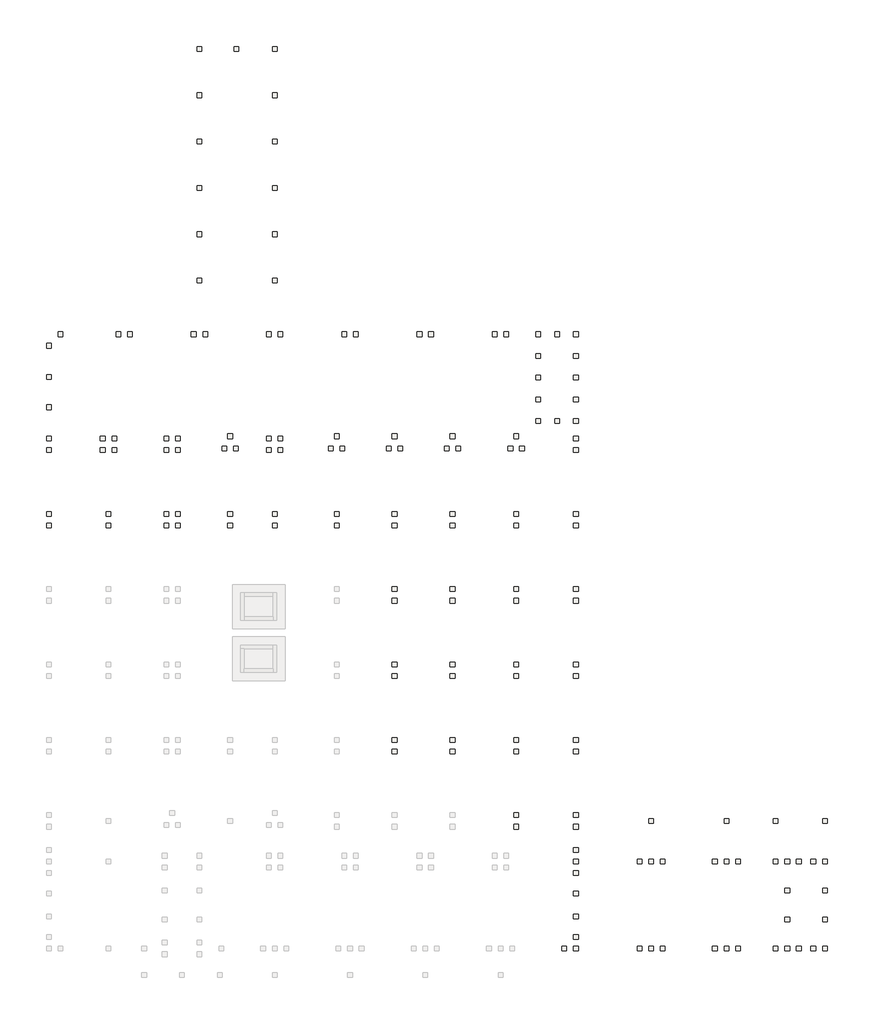
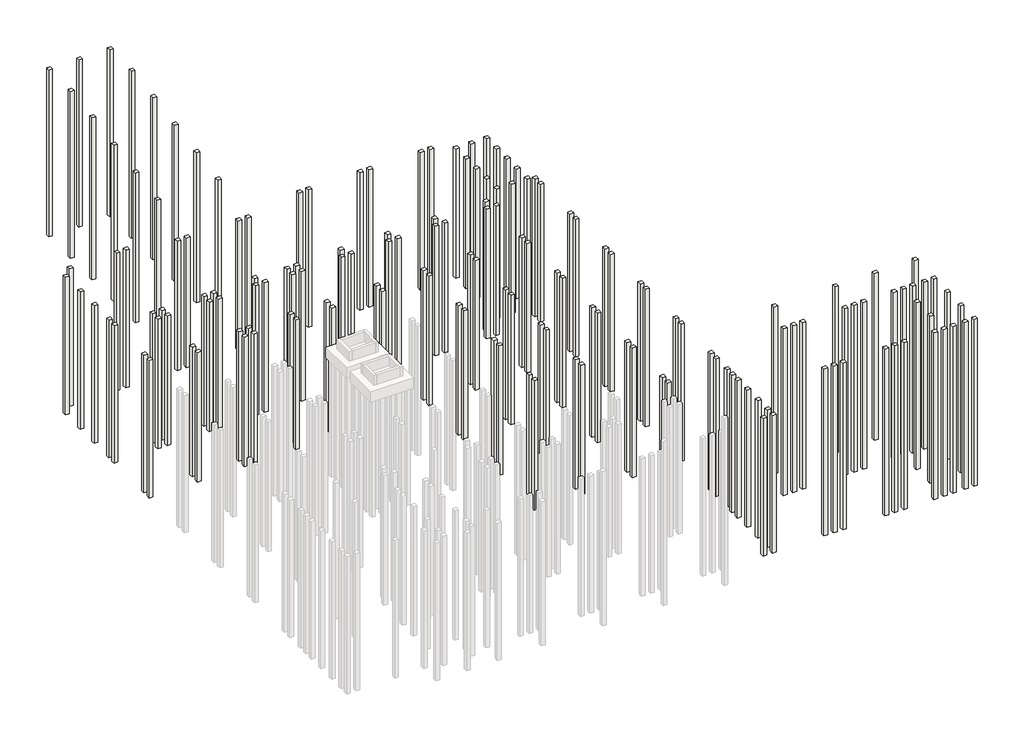
# Not in any storey, part 2 of 2: 160 slabs.
# Revit data of these elements (continued)
# Element 105 (IfcSlab, "NLRS_17_SFO_TLB_funderingspaal geheid beton prefab-AV-MMBPC_gen_rsf : heipaal beton prefab_gen__bxh 400x400")
#   IfcGUID = "3loy75XKz2Rw4dS8JWiatE"
#   Slanted Angle = 0.00°
#   NLRS_S_draagvermogen_trek = 0.00 kN
#   NLRS_S_draagvermogen_druk = 0.00 kN
#   Angle = 0.00°
#   IsExternal = yes
#   LoadBearing = yes
#   Slanted = 0
#   Phase Created = NLRS_nieuw
#   Materials on its faces: "NLRS_f2_beton prefab_gen_rsf"
# Element 106 (IfcSlab, "NLRS_17_SFO_TLB_funderingspaal geheid beton prefab-AV-MMBPC_gen_rsf : heipaal beton prefab_gen__bxh 400x400")
#   IfcGUID = "3loy75XKz2Rw4dS8JWiatC"
#   Slanted Angle = 0.00°
#   NLRS_S_draagvermogen_trek = 0.00 kN
#   NLRS_S_draagvermogen_druk = 0.00 kN
#   Angle = 0.00°
#   IsExternal = yes
#   LoadBearing = yes
#   Slanted = 0
#   Phase Created = NLRS_nieuw
#   Materials on its faces: "NLRS_f2_beton prefab_gen_rsf"
# Element 107 (IfcSlab, "NLRS_17_SFO_TLB_funderingspaal geheid beton prefab-AV-MMBPC_gen_rsf : heipaal beton prefab_gen__bxh 400x400")
#   IfcGUID = "3loy75XKz2Rw4dS8JWiatv"
#   Slanted Angle = 0.00°
#   NLRS_S_draagvermogen_trek = 0.00 kN
#   NLRS_S_draagvermogen_druk = 0.00 kN
#   Angle = 0.00°
#   IsExternal = yes
#   LoadBearing = yes
#   Slanted = 0
#   Phase Created = NLRS_nieuw
#   Materials on its faces: "NLRS_f2_beton prefab_gen_rsf"
# Element 108 (IfcSlab, "NLRS_17_SFO_TLB_funderingspaal geheid beton prefab-AV-MMBPC_gen_rsf : heipaal beton prefab_gen__bxh 400x400")
#   IfcGUID = "3loy75XKz2Rw4dS8JWiat$"
#   Slanted Angle = 0.00°
#   NLRS_S_draagvermogen_trek = 0.00 kN
#   NLRS_S_draagvermogen_druk = 0.00 kN
#   Angle = 0.00°
#   IsExternal = yes
#   LoadBearing = yes
#   Slanted = 0
#   Phase Created = NLRS_nieuw
#   Materials on its faces: "NLRS_f2_beton prefab_gen_rsf"
# Element 109 (IfcSlab, "NLRS_17_SFO_TLB_funderingspaal geheid beton prefab-AV-MMBPC_gen_rsf : heipaal beton prefab_gen__bxh 400x400")
#   IfcGUID = "3loy75XKz2Rw4dS8JWiaEQ"
#   Slanted Angle = 0.00°
#   NLRS_S_draagvermogen_trek = 0.00 kN
#   NLRS_S_draagvermogen_druk = 0.00 kN
#   Angle = 0.00°
#   IsExternal = yes
#   LoadBearing = yes
#   Slanted = 0
#   Phase Created = NLRS_nieuw
#   Materials on its faces: "NLRS_f2_beton prefab_gen_rsf"
# Element 110 (IfcSlab, "NLRS_17_SFO_TLB_funderingspaal geheid beton prefab-AV-MMBPC_gen_rsf : heipaal beton prefab_gen__bxh 400x400")
#   IfcGUID = "3loy75XKz2Rw4dS8JWiaEW"
#   Slanted Angle = 0.00°
#   NLRS_S_draagvermogen_trek = 0.00 kN
#   NLRS_S_draagvermogen_druk = 0.00 kN
#   Angle = 0.00°
#   IsExternal = yes
#   LoadBearing = yes
#   Slanted = 0
#   Phase Created = NLRS_nieuw
#   Materials on its faces: "NLRS_f2_beton prefab_gen_rsf"
# Element 111 (IfcSlab, "NLRS_17_SFO_TLB_funderingspaal geheid beton prefab-AV-MMBPC_gen_rsf : heipaal beton prefab_gen__bxh 400x400")
#   IfcGUID = "3loy75XKz2Rw4dS8JWia10"
#   Slanted Angle = 0.00°
#   NLRS_S_draagvermogen_trek = 0.00 kN
#   NLRS_S_draagvermogen_druk = 0.00 kN
#   Angle = 0.00°
#   IsExternal = yes
#   LoadBearing = yes
#   Slanted = 0
#   Phase Created = NLRS_nieuw
#   Materials on its faces: "NLRS_f2_beton prefab_gen_rsf"
# Element 112 (IfcSlab, "NLRS_17_SFO_TLB_funderingspaal geheid beton prefab-AV-MMBPC_gen_rsf : heipaal beton prefab_gen__bxh 400x400")
#   IfcGUID = "3loy75XKz2Rw4dS8JWia16"
#   Slanted Angle = 0.00°
#   NLRS_S_draagvermogen_trek = 0.00 kN
#   NLRS_S_draagvermogen_druk = 0.00 kN
#   Angle = 0.00°
#   IsExternal = yes
#   LoadBearing = yes
#   Slanted = 0
#   Phase Created = NLRS_nieuw
#   Materials on its faces: "NLRS_f2_beton prefab_gen_rsf"
# Element 113 (IfcSlab, "NLRS_17_SFO_TLB_funderingspaal geheid beton prefab-AV-MMBPC_gen_rsf : heipaal beton prefab_gen__bxh 400x400")
#   IfcGUID = "3loy75XKz2Rw4dS8JWia1p"
#   Slanted Angle = 0.00°
#   NLRS_S_draagvermogen_trek = 0.00 kN
#   NLRS_S_draagvermogen_druk = 0.00 kN
#   Angle = 0.00°
#   IsExternal = yes
#   LoadBearing = yes
#   Slanted = 0
#   Phase Created = NLRS_nieuw
#   Materials on its faces: "NLRS_f2_beton prefab_gen_rsf"
# Element 114 (IfcSlab, "NLRS_17_SFO_TLB_funderingspaal geheid beton prefab-AV-MMBPC_gen_rsf : heipaal beton prefab_gen__bxh 400x400")
#   IfcGUID = "3loy75XKz2Rw4dS8JWia1n"
#   Slanted Angle = 0.00°
#   NLRS_S_draagvermogen_trek = 0.00 kN
#   NLRS_S_draagvermogen_druk = 0.00 kN
#   Angle = 0.00°
#   IsExternal = yes
#   LoadBearing = yes
#   Slanted = 0
#   Phase Created = NLRS_nieuw
#   Materials on its faces: "NLRS_f2_beton prefab_gen_rsf"
# Element 115 (IfcSlab, "NLRS_17_SFO_TLB_funderingspaal geheid beton prefab-AV-MMBPC_gen_rsf : heipaal beton prefab_gen__bxh 400x400")
#   IfcGUID = "3loy75XKz2Rw4dS8JWia5x"
#   Slanted Angle = 0.00°
#   NLRS_S_draagvermogen_trek = 0.00 kN
#   NLRS_S_draagvermogen_druk = 0.00 kN
#   Angle = 0.00°
#   IsExternal = yes
#   LoadBearing = yes
#   Slanted = 0
#   Phase Created = NLRS_nieuw
#   Materials on its faces: "NLRS_f2_beton prefab_gen_rsf"
# Element 116 (IfcSlab, "NLRS_17_SFO_TLB_funderingspaal geheid beton prefab-AV-MMBPC_gen_rsf : heipaal beton prefab_gen__bxh 400x400")
#   IfcGUID = "3loy75XKz2Rw4dS8JWia4Y"
#   Slanted Angle = 0.00°
#   NLRS_S_draagvermogen_trek = 0.00 kN
#   NLRS_S_draagvermogen_druk = 0.00 kN
#   Angle = 0.00°
#   IsExternal = yes
#   LoadBearing = yes
#   Slanted = 0
#   Phase Created = NLRS_nieuw
#   Materials on its faces: "NLRS_f2_beton prefab_gen_rsf"
# Element 117 (IfcSlab, "NLRS_17_SFO_TLB_funderingspaal geheid beton prefab-AV-MMBPC_gen_rsf : heipaal beton prefab_gen__bxh 400x400")
#   IfcGUID = "3loy75XKz2Rw4dS8JWia4W"
#   Slanted Angle = 0.00°
#   NLRS_S_draagvermogen_trek = 0.00 kN
#   NLRS_S_draagvermogen_druk = 0.00 kN
#   Angle = 0.00°
#   IsExternal = yes
#   LoadBearing = yes
#   Slanted = 0
#   Phase Created = NLRS_nieuw
#   Materials on its faces: "NLRS_f2_beton prefab_gen_rsf"
# Element 118 (IfcSlab, "NLRS_17_SFO_TLB_funderingspaal geheid beton prefab-AV-MMBPC_gen_rsf : heipaal beton prefab_gen__bxh 400x400")
#   IfcGUID = "1JrsWFyZX6xPuD52juGVxa"
#   Slanted Angle = 0.00°
#   NLRS_S_draagvermogen_trek = 0.00 kN
#   NLRS_S_draagvermogen_druk = 0.00 kN
#   Angle = 0.00°
#   IsExternal = yes
#   LoadBearing = yes
#   Slanted = 0
#   Phase Created = NLRS_nieuw
#   Materials on its faces: "NLRS_f2_beton prefab_gen_rsf"
# Element 119 (IfcSlab, "NLRS_17_SFO_TLB_funderingspaal geheid beton prefab-AV-MMBPC_gen_rsf : heipaal beton prefab_gen__bxh 400x400")
#   IfcGUID = "1JrsWFyZX6xPuD52juGVvn"
#   Slanted Angle = 0.00°
#   NLRS_S_draagvermogen_trek = 0.00 kN
#   NLRS_S_draagvermogen_druk = 0.00 kN
#   Angle = 0.00°
#   IsExternal = yes
#   LoadBearing = yes
#   Slanted = 0
#   Phase Created = NLRS_nieuw
#   Materials on its faces: "NLRS_f2_beton prefab_gen_rsf"
# Element 120 (IfcSlab, "NLRS_17_SFO_TLB_funderingspaal geheid beton prefab-AV-MMBPC_gen_rsf : heipaal beton prefab_gen__bxh 400x400")
#   IfcGUID = "1JrsWFyZX6xPuD52juGVv2"
#   Slanted Angle = 0.00°
#   NLRS_S_draagvermogen_trek = 0.00 kN
#   NLRS_S_draagvermogen_druk = 0.00 kN
#   Angle = 0.00°
#   IsExternal = yes
#   LoadBearing = yes
#   Slanted = 0
#   Phase Created = NLRS_nieuw
#   Materials on its faces: "NLRS_f2_beton prefab_gen_rsf"
# Element 121 (IfcSlab, "NLRS_17_SFO_TLB_funderingspaal geheid beton prefab-AV-MMBPC_gen_rsf : heipaal beton prefab_gen__bxh 400x400")
#   IfcGUID = "1JrsWFyZX6xPuD52juGV_f"
#   Slanted Angle = 0.00°
#   NLRS_S_draagvermogen_trek = 0.00 kN
#   NLRS_S_draagvermogen_druk = 0.00 kN
#   Angle = 0.00°
#   IsExternal = yes
#   LoadBearing = yes
#   Slanted = 0
#   Phase Created = NLRS_nieuw
#   Materials on its faces: "NLRS_f2_beton prefab_gen_rsf"
# Element 122 (IfcSlab, "NLRS_17_SFO_TLB_funderingspaal geheid beton prefab-AV-MMBPC_gen_rsf : heipaal beton prefab_gen__bxh 400x400")
#   IfcGUID = "1JrsWFyZX6xPuD52juGV_d"
#   Slanted Angle = 0.00°
#   NLRS_S_draagvermogen_trek = 0.00 kN
#   NLRS_S_draagvermogen_druk = 0.00 kN
#   Angle = 0.00°
#   IsExternal = yes
#   LoadBearing = yes
#   Slanted = 0
#   Phase Created = NLRS_nieuw
#   Materials on its faces: "NLRS_f2_beton prefab_gen_rsf"
# Element 123 (IfcSlab, "NLRS_17_SFO_TLB_funderingspaal geheid beton prefab-AV-MMBPC_gen_rsf : heipaal beton prefab_gen__bxh 400x400")
#   IfcGUID = "1JrsWFyZX6xPuD52juGV_b"
#   Slanted Angle = 0.00°
#   NLRS_S_draagvermogen_trek = 0.00 kN
#   NLRS_S_draagvermogen_druk = 0.00 kN
#   Angle = 0.00°
#   IsExternal = yes
#   LoadBearing = yes
#   Slanted = 0
#   Phase Created = NLRS_nieuw
#   Materials on its faces: "NLRS_f2_beton prefab_gen_rsf"
# Element 124 (IfcSlab, "NLRS_17_SFO_TLB_funderingspaal geheid beton prefab-AV-MMBPC_gen_rsf : heipaal beton prefab_gen__bxh 400x400")
#   IfcGUID = "1JrsWFyZX6xPuD52juGV_G"
#   Slanted Angle = 0.00°
#   NLRS_S_draagvermogen_trek = 0.00 kN
#   NLRS_S_draagvermogen_druk = 0.00 kN
#   Angle = 0.00°
#   IsExternal = yes
#   LoadBearing = yes
#   Slanted = 0
#   Phase Created = NLRS_nieuw
#   Materials on its faces: "NLRS_f2_beton prefab_gen_rsf"
# Element 125 (IfcSlab, "NLRS_17_SFO_TLB_funderingspaal geheid beton prefab-AV-MMBPC_gen_rsf : heipaal beton prefab_gen__bxh 400x400")
#   IfcGUID = "1JrsWFyZX6xPuD52juGV_E"
#   Slanted Angle = 0.00°
#   NLRS_S_draagvermogen_trek = 0.00 kN
#   NLRS_S_draagvermogen_druk = 0.00 kN
#   Angle = 0.00°
#   IsExternal = yes
#   LoadBearing = yes
#   Slanted = 0
#   Phase Created = NLRS_nieuw
#   Materials on its faces: "NLRS_f2_beton prefab_gen_rsf"
# Element 126 (IfcSlab, "NLRS_17_SFO_TLB_funderingspaal geheid beton prefab-AV-MMBPC_gen_rsf : heipaal beton prefab_gen__bxh 400x400")
#   IfcGUID = "1JrsWFyZX6xPuD52juGV_C"
#   Slanted Angle = 0.00°
#   NLRS_S_draagvermogen_trek = 0.00 kN
#   NLRS_S_draagvermogen_druk = 0.00 kN
#   Angle = 0.00°
#   IsExternal = yes
#   LoadBearing = yes
#   Slanted = 0
#   Phase Created = NLRS_nieuw
#   Materials on its faces: "NLRS_f2_beton prefab_gen_rsf"
# Element 127 (IfcSlab, "NLRS_17_SFO_TLB_funderingspaal geheid beton prefab-AV-MMBPC_gen_rsf : heipaal beton prefab_gen__bxh 400x400")
#   IfcGUID = "1JrsWFyZX6xPuD52juGV_A"
#   Slanted Angle = 0.00°
#   NLRS_S_draagvermogen_trek = 0.00 kN
#   NLRS_S_draagvermogen_druk = 0.00 kN
#   Angle = 0.00°
#   IsExternal = yes
#   LoadBearing = yes
#   Slanted = 0
#   Phase Created = NLRS_nieuw
#   Materials on its faces: "NLRS_f2_beton prefab_gen_rsf"
# Element 128 (IfcSlab, "NLRS_17_SFO_TLB_funderingspaal geheid beton prefab-AV-MMBPC_gen_rsf : heipaal beton prefab_gen__bxh 400x400")
#   IfcGUID = "1JrsWFyZX6xPuD52juGV_8"
#   Slanted Angle = 0.00°
#   NLRS_S_draagvermogen_trek = 0.00 kN
#   NLRS_S_draagvermogen_druk = 0.00 kN
#   Angle = 0.00°
#   IsExternal = yes
#   LoadBearing = yes
#   Slanted = 0
#   Phase Created = NLRS_nieuw
#   Materials on its faces: "NLRS_f2_beton prefab_gen_rsf"
# Element 129 (IfcSlab, "NLRS_17_SFO_TLB_funderingspaal geheid beton prefab-AV-MMBPC_gen_rsf : heipaal beton prefab_gen__bxh 400x400")
#   IfcGUID = "1JrsWFyZX6xPuD52juGV_6"
#   Slanted Angle = 0.00°
#   NLRS_S_draagvermogen_trek = 0.00 kN
#   NLRS_S_draagvermogen_druk = 0.00 kN
#   Angle = 0.00°
#   IsExternal = yes
#   LoadBearing = yes
#   Slanted = 0
#   Phase Created = NLRS_nieuw
#   Materials on its faces: "NLRS_f2_beton prefab_gen_rsf"
# Element 130 (IfcSlab, "NLRS_17_SFO_TLB_funderingspaal geheid beton prefab-AV-MMBPC_gen_rsf : heipaal beton prefab_gen__bxh 400x400")
#   IfcGUID = "1JrsWFyZX6xPuD52juGV$T"
#   Slanted Angle = 0.00°
#   NLRS_S_draagvermogen_trek = 0.00 kN
#   NLRS_S_draagvermogen_druk = 0.00 kN
#   Angle = 0.00°
#   IsExternal = yes
#   LoadBearing = yes
#   Slanted = 0
#   Phase Created = NLRS_nieuw
#   Materials on its faces: "NLRS_f2_beton prefab_gen_rsf"
# Element 131 (IfcSlab, "NLRS_17_SFO_TLB_funderingspaal geheid beton prefab-AV-MMBPC_gen_rsf : heipaal beton prefab_gen__bxh 400x400")
#   IfcGUID = "1JrsWFyZX6xPuD52juGV$G"
#   Slanted Angle = 0.00°
#   NLRS_S_draagvermogen_trek = 0.00 kN
#   NLRS_S_draagvermogen_druk = 0.00 kN
#   Angle = 0.00°
#   IsExternal = yes
#   LoadBearing = yes
#   Slanted = 0
#   Phase Created = NLRS_nieuw
#   Materials on its faces: "NLRS_f2_beton prefab_gen_rsf"
# Element 132 (IfcSlab, "NLRS_17_SFO_TLB_funderingspaal geheid beton prefab-AV-MMBPC_gen_rsf : heipaal beton prefab_gen__bxh 400x400")
#   IfcGUID = "1JrsWFyZX6xPuD52juGVyj"
#   Slanted Angle = 0.00°
#   NLRS_S_draagvermogen_trek = 0.00 kN
#   NLRS_S_draagvermogen_druk = 0.00 kN
#   Angle = 0.00°
#   IsExternal = yes
#   LoadBearing = yes
#   Slanted = 0
#   Phase Created = NLRS_nieuw
#   Materials on its faces: "NLRS_f2_beton prefab_gen_rsf"
# Element 133 (IfcSlab, "NLRS_17_SFO_TLB_funderingspaal geheid beton prefab-AV-MMBPC_gen_rsf : heipaal beton prefab_gen__bxh 400x400")
#   IfcGUID = "1JrsWFyZX6xPuD52juGVy1"
#   Slanted Angle = 0.00°
#   NLRS_S_draagvermogen_trek = 0.00 kN
#   NLRS_S_draagvermogen_druk = 0.00 kN
#   Angle = 0.00°
#   IsExternal = yes
#   LoadBearing = yes
#   Slanted = 0
#   Phase Created = NLRS_nieuw
#   Materials on its faces: "NLRS_f2_beton prefab_gen_rsf"
# Element 134 (IfcSlab, "NLRS_17_SFO_TLB_funderingspaal geheid beton prefab-AV-MMBPC_gen_rsf : heipaal beton prefab_gen__bxh 400x400")
#   IfcGUID = "1JrsWFyZX6xPuD52juGVz$"
#   Slanted Angle = 0.00°
#   NLRS_S_draagvermogen_trek = 0.00 kN
#   NLRS_S_draagvermogen_druk = 0.00 kN
#   Angle = 0.00°
#   IsExternal = yes
#   LoadBearing = yes
#   Slanted = 0
#   Phase Created = NLRS_nieuw
#   Materials on its faces: "NLRS_f2_beton prefab_gen_rsf"
# Element 135 (IfcSlab, "NLRS_17_SFO_TLB_funderingspaal geheid beton prefab-AV-MMBPC_gen_rsf : heipaal beton prefab_gen__bxh 400x400")
#   IfcGUID = "1JrsWFyZX6xPuD52juGVzz"
#   Slanted Angle = 0.00°
#   NLRS_S_draagvermogen_trek = 0.00 kN
#   NLRS_S_draagvermogen_druk = 0.00 kN
#   Angle = 0.00°
#   IsExternal = yes
#   LoadBearing = yes
#   Slanted = 0
#   Phase Created = NLRS_nieuw
#   Materials on its faces: "NLRS_f2_beton prefab_gen_rsf"
# Element 136 (IfcSlab, "NLRS_17_SFO_TLB_funderingspaal geheid beton prefab-AV-MMBPC_gen_rsf : heipaal beton prefab_gen__bxh 400x400")
#   IfcGUID = "1JrsWFyZX6xPuD52juGVzI"
#   Slanted Angle = 0.00°
#   NLRS_S_draagvermogen_trek = 0.00 kN
#   NLRS_S_draagvermogen_druk = 0.00 kN
#   Angle = 0.00°
#   IsExternal = yes
#   LoadBearing = yes
#   Slanted = 0
#   Phase Created = NLRS_nieuw
#   Materials on its faces: "NLRS_f2_beton prefab_gen_rsf"
# Element 137 (IfcSlab, "NLRS_17_SFO_TLB_funderingspaal geheid beton prefab-AV-MMBPC_gen_rsf : heipaal beton prefab_gen__bxh 400x400")
#   IfcGUID = "1JrsWFyZX6xPuD52juGVz7"
#   Slanted Angle = 0.00°
#   NLRS_S_draagvermogen_trek = 0.00 kN
#   NLRS_S_draagvermogen_druk = 0.00 kN
#   Angle = 0.00°
#   IsExternal = yes
#   LoadBearing = yes
#   Slanted = 0
#   Phase Created = NLRS_nieuw
#   Materials on its faces: "NLRS_f2_beton prefab_gen_rsf"
# Element 138 (IfcSlab, "NLRS_17_SFO_TLB_funderingspaal geheid beton prefab-AV-MMBPC_gen_rsf : heipaal beton prefab_gen__bxh 400x400")
#   IfcGUID = "1JrsWFyZX6xPuD52juGVog"
#   Slanted Angle = 0.00°
#   NLRS_S_draagvermogen_trek = 0.00 kN
#   NLRS_S_draagvermogen_druk = 0.00 kN
#   Angle = 0.00°
#   IsExternal = yes
#   LoadBearing = yes
#   Slanted = 0
#   Phase Created = NLRS_nieuw
#   Materials on its faces: "NLRS_f2_beton prefab_gen_rsf"
# Element 139 (IfcSlab, "NLRS_17_SFO_TLB_funderingspaal geheid beton prefab-AV-MMBPC_gen_rsf : heipaal beton prefab_gen__bxh 400x400")
#   IfcGUID = "1JrsWFyZX6xPuD52juGVoe"
#   Slanted Angle = 0.00°
#   NLRS_S_draagvermogen_trek = 0.00 kN
#   NLRS_S_draagvermogen_druk = 0.00 kN
#   Angle = 0.00°
#   IsExternal = yes
#   LoadBearing = yes
#   Slanted = 0
#   Phase Created = NLRS_nieuw
#   Materials on its faces: "NLRS_f2_beton prefab_gen_rsf"
# Element 140 (IfcSlab, "NLRS_17_SFO_TLB_funderingspaal geheid beton prefab-AV-MMBPC_gen_rsf : heipaal beton prefab_gen__bxh 400x400")
#   IfcGUID = "1JrsWFyZX6xPuD52juGVpj"
#   Slanted Angle = 0.00°
#   NLRS_S_draagvermogen_trek = 0.00 kN
#   NLRS_S_draagvermogen_druk = 0.00 kN
#   Angle = 0.00°
#   IsExternal = yes
#   LoadBearing = yes
#   Slanted = 0
#   Phase Created = NLRS_nieuw
#   Materials on its faces: "NLRS_f2_beton prefab_gen_rsf"
# Element 141 (IfcSlab, "NLRS_17_SFO_TLB_funderingspaal geheid beton prefab-AV-MMBPC_gen_rsf : heipaal beton prefab_gen__bxh 400x400")
#   IfcGUID = "1JrsWFyZX6xPuD52juGVph"
#   Slanted Angle = 0.00°
#   NLRS_S_draagvermogen_trek = 0.00 kN
#   NLRS_S_draagvermogen_druk = 0.00 kN
#   Angle = 0.00°
#   IsExternal = yes
#   LoadBearing = yes
#   Slanted = 0
#   Phase Created = NLRS_nieuw
#   Materials on its faces: "NLRS_f2_beton prefab_gen_rsf"
# Element 142 (IfcSlab, "NLRS_17_SFO_TLB_funderingspaal geheid beton prefab-AV-MMBPC_gen_rsf : heipaal beton prefab_gen__bxh 400x400")
#   IfcGUID = "1JrsWFyZX6xPuD52juGVp8"
#   Slanted Angle = 0.00°
#   NLRS_S_draagvermogen_trek = 0.00 kN
#   NLRS_S_draagvermogen_druk = 0.00 kN
#   Angle = 0.00°
#   IsExternal = yes
#   LoadBearing = yes
#   Slanted = 0
#   Phase Created = NLRS_nieuw
#   Materials on its faces: "NLRS_f2_beton prefab_gen_rsf"
# Element 143 (IfcSlab, "NLRS_17_SFO_TLB_funderingspaal geheid beton prefab-AV-MMBPC_gen_rsf : heipaal beton prefab_gen__bxh 400x400")
#   IfcGUID = "1JrsWFyZX6xPuD52juGVp6"
#   Slanted Angle = 0.00°
#   NLRS_S_draagvermogen_trek = 0.00 kN
#   NLRS_S_draagvermogen_druk = 0.00 kN
#   Angle = 0.00°
#   IsExternal = yes
#   LoadBearing = yes
#   Slanted = 0
#   Phase Created = NLRS_nieuw
#   Materials on its faces: "NLRS_f2_beton prefab_gen_rsf"
# Element 144 (IfcSlab, "NLRS_17_SFO_TLB_funderingspaal geheid beton prefab-AV-MMBPC_gen_rsf : heipaal beton prefab_gen__bxh 400x400")
#   IfcGUID = "1JrsWFyZX6xPuD52juGVmn"
#   Slanted Angle = 0.00°
#   NLRS_S_draagvermogen_trek = 0.00 kN
#   NLRS_S_draagvermogen_druk = 0.00 kN
#   Angle = 0.00°
#   IsExternal = yes
#   LoadBearing = yes
#   Slanted = 0
#   Phase Created = NLRS_nieuw
#   Materials on its faces: "NLRS_f2_beton prefab_gen_rsf"
# Element 145 (IfcSlab, "NLRS_17_SFO_TLB_funderingspaal geheid beton prefab-AV-MMBPC_gen_rsf : heipaal beton prefab_gen__bxh 400x400")
#   IfcGUID = "1JrsWFyZX6xPuD52juGVm6"
#   Slanted Angle = 0.00°
#   NLRS_S_draagvermogen_trek = 0.00 kN
#   NLRS_S_draagvermogen_druk = 0.00 kN
#   Angle = 0.00°
#   IsExternal = yes
#   LoadBearing = yes
#   Slanted = 0
#   Phase Created = NLRS_nieuw
#   Materials on its faces: "NLRS_f2_beton prefab_gen_rsf"
# Element 146 (IfcSlab, "NLRS_17_SFO_TLB_funderingspaal geheid beton prefab-AV-MMBPC_gen_rsf : heipaal beton prefab_gen__bxh 400x400")
#   IfcGUID = "1JrsWFyZX6xPuD52juGVnx"
#   Slanted Angle = 0.00°
#   NLRS_S_draagvermogen_trek = 0.00 kN
#   NLRS_S_draagvermogen_druk = 0.00 kN
#   Angle = 0.00°
#   IsExternal = yes
#   LoadBearing = yes
#   Slanted = 0
#   Phase Created = NLRS_nieuw
#   Materials on its faces: "NLRS_f2_beton prefab_gen_rsf"
# Element 147 (IfcSlab, "NLRS_17_SFO_TLB_funderingspaal geheid beton prefab-AV-MMBPC_gen_rsf : heipaal beton prefab_gen__bxh 400x400")
#   IfcGUID = "1JrsWFyZX6xPuD52juGVnv"
#   Slanted Angle = 0.00°
#   NLRS_S_draagvermogen_trek = 0.00 kN
#   NLRS_S_draagvermogen_druk = 0.00 kN
#   Angle = 0.00°
#   IsExternal = yes
#   LoadBearing = yes
#   Slanted = 0
#   Phase Created = NLRS_nieuw
#   Materials on its faces: "NLRS_f2_beton prefab_gen_rsf"
# Element 148 (IfcSlab, "NLRS_17_SFO_TLB_funderingspaal geheid beton prefab-AV-MMBPC_gen_rsf : heipaal beton prefab_gen__bxh 400x400")
#   IfcGUID = "3aMdMHoe12P9KDGPyaIhq7"
#   Slanted Angle = 0.00°
#   NLRS_S_draagvermogen_trek = 0.00 kN
#   NLRS_S_draagvermogen_druk = 0.00 kN
#   Angle = 0.00°
#   IsExternal = yes
#   LoadBearing = yes
#   Slanted = 0
#   Phase Created = NLRS_nieuw
#   Materials on its faces: "NLRS_f2_beton prefab_gen_rsf"
# Element 149 (IfcSlab, "NLRS_17_SFO_TLB_funderingspaal geheid beton prefab-AV-MMBPC_gen_rsf : heipaal beton prefab_gen__bxh 400x400")
#   IfcGUID = "3aMdMHoe12P9KDGPyaIhqK"
#   Slanted Angle = 0.00°
#   NLRS_S_draagvermogen_trek = 0.00 kN
#   NLRS_S_draagvermogen_druk = 0.00 kN
#   Angle = 0.00°
#   IsExternal = yes
#   LoadBearing = yes
#   Slanted = 0
#   Phase Created = NLRS_nieuw
#   Materials on its faces: "NLRS_f2_beton prefab_gen_rsf"
# Element 150 (IfcSlab, "NLRS_17_SFO_TLB_funderingspaal geheid beton prefab-AV-MMBPC_gen_rsf : heipaal beton prefab_gen__bxh 400x400")
#   IfcGUID = "3aMdMHoe12P9KDGPyaIhth"
#   Slanted Angle = 0.00°
#   NLRS_S_draagvermogen_trek = 0.00 kN
#   NLRS_S_draagvermogen_druk = 0.00 kN
#   Angle = 0.00°
#   IsExternal = yes
#   LoadBearing = yes
#   Slanted = 0
#   Phase Created = NLRS_nieuw
#   Materials on its faces: "NLRS_f2_beton prefab_gen_rsf"
# Element 151 (IfcSlab, "NLRS_17_SFO_TLB_funderingspaal geheid beton prefab-AV-MMBPC_gen_rsf : heipaal beton prefab_gen__bxh 400x400")
#   IfcGUID = "3aMdMHoe12P9KDGPyaIht6"
#   Slanted Angle = 0.00°
#   NLRS_S_draagvermogen_trek = 0.00 kN
#   NLRS_S_draagvermogen_druk = 0.00 kN
#   Angle = 0.00°
#   IsExternal = yes
#   LoadBearing = yes
#   Slanted = 0
#   Phase Created = NLRS_nieuw
#   Materials on its faces: "NLRS_f2_beton prefab_gen_rsf"
# Element 152 (IfcSlab, "NLRS_17_SFO_TLB_funderingspaal geheid beton prefab-AV-MMBPC_gen_rsf : heipaal beton prefab_gen__bxh 400x400")
#   IfcGUID = "3aMdMHoe12P9KDGPyaIhtP"
#   Slanted Angle = 0.00°
#   NLRS_S_draagvermogen_trek = 0.00 kN
#   NLRS_S_draagvermogen_druk = 0.00 kN
#   Angle = 0.00°
#   IsExternal = yes
#   LoadBearing = yes
#   Slanted = 0
#   Phase Created = NLRS_nieuw
#   Materials on its faces: "NLRS_f2_beton prefab_gen_rsf"
# Element 153 (IfcSlab, "NLRS_17_SFO_TLB_funderingspaal geheid beton prefab-AV-MMBPC_gen_rsf : heipaal beton prefab_gen__bxh 400x400")
#   IfcGUID = "3aMdMHoe12P9KDGPyaIhsw"
#   Slanted Angle = 0.00°
#   NLRS_S_draagvermogen_trek = 0.00 kN
#   NLRS_S_draagvermogen_druk = 0.00 kN
#   Angle = 0.00°
#   IsExternal = yes
#   LoadBearing = yes
#   Slanted = 0
#   Phase Created = NLRS_nieuw
#   Materials on its faces: "NLRS_f2_beton prefab_gen_rsf"
# Element 154 (IfcSlab, "NLRS_17_SFO_TLB_funderingspaal geheid beton prefab-AV-MMBPC_gen_rsf : heipaal beton prefab_gen__bxh 400x400")
#   IfcGUID = "3aMdMHoe12P9KDGPyaIhxf"
#   Slanted Angle = 0.00°
#   NLRS_S_draagvermogen_trek = 0.00 kN
#   NLRS_S_draagvermogen_druk = 0.00 kN
#   Angle = 0.00°
#   IsExternal = yes
#   LoadBearing = yes
#   Slanted = 0
#   Phase Created = NLRS_nieuw
#   Materials on its faces: "NLRS_f2_beton prefab_gen_rsf"
# Element 155 (IfcSlab, "NLRS_17_SFO_TLB_funderingspaal geheid beton prefab-AV-MMBPC_gen_rsf : heipaal beton prefab_gen__bxh 400x400")
#   IfcGUID = "3aMdMHoe12P9KDGPyaIhsp"
#   Slanted Angle = 0.00°
#   NLRS_S_draagvermogen_trek = 0.00 kN
#   NLRS_S_draagvermogen_druk = 0.00 kN
#   Angle = 0.00°
#   IsExternal = yes
#   LoadBearing = yes
#   Slanted = 0
#   Phase Created = NLRS_nieuw
#   Materials on its faces: "NLRS_f2_beton prefab_gen_rsf"
# Element 156 (IfcSlab, "NLRS_17_SFO_TLB_funderingspaal geheid beton prefab-AV-MMBPC_gen_rsf : heipaal beton prefab_gen__bxh 400x400")
#   IfcGUID = "3aMdMHoe12P9KDGPyaIhxd"
#   Slanted Angle = 0.00°
#   NLRS_S_draagvermogen_trek = 0.00 kN
#   NLRS_S_draagvermogen_druk = 0.00 kN
#   Angle = 0.00°
#   IsExternal = yes
#   LoadBearing = yes
#   Slanted = 0
#   Phase Created = NLRS_nieuw
#   Materials on its faces: "NLRS_f2_beton prefab_gen_rsf"
# Element 157 (IfcSlab, "NLRS_17_SFO_TLB_funderingspaal geheid beton prefab-AV-MMBPC_gen_rsf : heipaal beton prefab_gen__bxh 400x400")
#   IfcGUID = "3aMdMHoe12P9KDGPyaIhs8"
#   Slanted Angle = 0.00°
#   NLRS_S_draagvermogen_trek = 0.00 kN
#   NLRS_S_draagvermogen_druk = 0.00 kN
#   Angle = 0.00°
#   IsExternal = yes
#   LoadBearing = yes
#   Slanted = 0
#   Phase Created = NLRS_nieuw
#   Materials on its faces: "NLRS_f2_beton prefab_gen_rsf"
# Element 158 (IfcSlab, "NLRS_17_SFO_TLB_funderingspaal geheid beton prefab-AV-MMBPC_gen_rsf : heipaal beton prefab_gen__bxh 400x400")
#   IfcGUID = "3aMdMHoe12P9KDGPyaIhxb"
#   Slanted Angle = 0.00°
#   NLRS_S_draagvermogen_trek = 0.00 kN
#   NLRS_S_draagvermogen_druk = 0.00 kN
#   Angle = 0.00°
#   IsExternal = yes
#   LoadBearing = yes
#   Slanted = 0
#   Phase Created = NLRS_nieuw
#   Materials on its faces: "NLRS_f2_beton prefab_gen_rsf"
# Element 159 (IfcSlab, "NLRS_17_SFO_TLB_funderingspaal geheid beton prefab-AV-MMBPC_gen_rsf : heipaal beton prefab_gen__bxh 400x400")
#   IfcGUID = "3aMdMHoe12P9KDGPyaIhs1"
#   Slanted Angle = 0.00°
#   NLRS_S_draagvermogen_trek = 0.00 kN
#   NLRS_S_draagvermogen_druk = 0.00 kN
#   Angle = 0.00°
#   IsExternal = yes
#   LoadBearing = yes
#   Slanted = 0
#   Phase Created = NLRS_nieuw
#   Materials on its faces: "NLRS_f2_beton prefab_gen_rsf"
# Element 160 (IfcSlab, "NLRS_17_SFO_TLB_funderingspaal geheid beton prefab-AV-MMBPC_gen_rsf : heipaal beton prefab_gen__bxh 400x400")
#   IfcGUID = "3aMdMHoe12P9KDGPyaIhxZ"
#   Slanted Angle = 0.00°
#   NLRS_S_draagvermogen_trek = 0.00 kN
#   NLRS_S_draagvermogen_druk = 0.00 kN
#   Angle = 0.00°
#   IsExternal = yes
#   LoadBearing = yes
#   Slanted = 0
#   Phase Created = NLRS_nieuw
#   Materials on its faces: "NLRS_f2_beton prefab_gen_rsf"
# Materials
#   "NLRS_f2_beton prefab_gen_rsf": class "F - Niet gebakken kunststeen", colour RGB 129 133 118, transparency 0, Keynote = "f2", Manufacturer = "Revit Standards Foundation", URL = "www.revitstandards.org", Description = "beton prefab", Cost = 0
